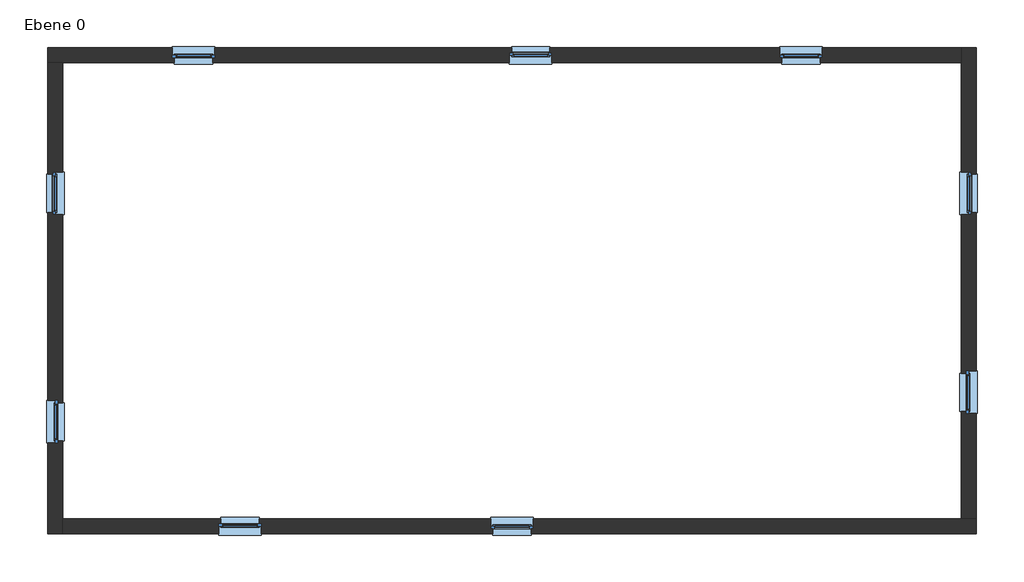
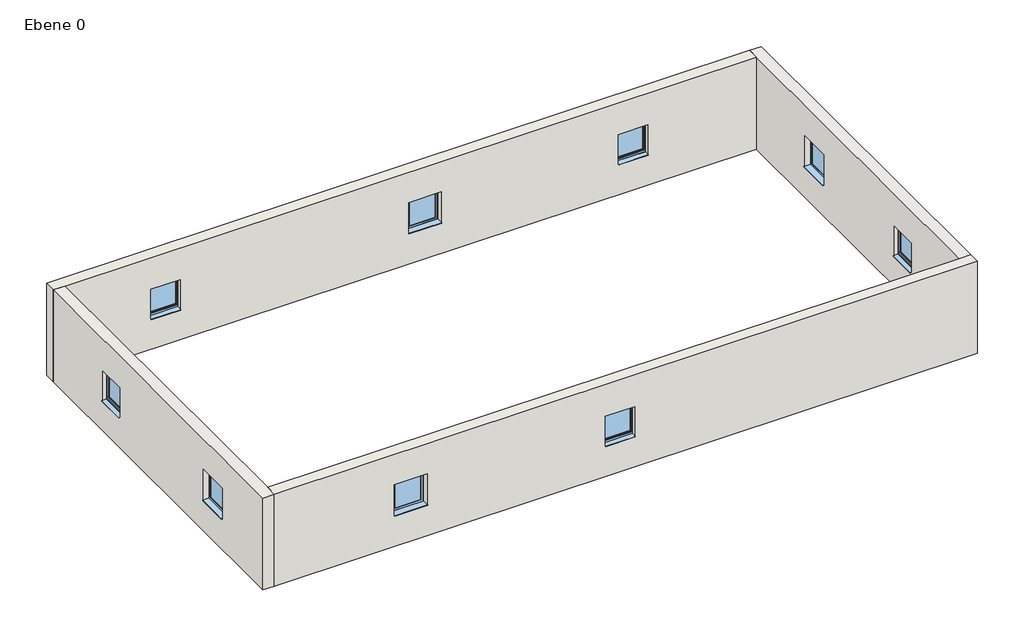
# One storey: 9 windows, 4 walls.
"""IFC4 building model written with IfcOpenShell, lengths in millimetres."""

import ifcopenshell
import ifcopenshell.guid

model = None  # the IFC model being written
_history = None  # IfcOwnerHistory: only IFC2X3 demands one
_inside = {}  # id of a spatial element -> (the spatial element, [elements in it])
_under = {}  # id of a project, library or spatial element -> (it, [spatial elements below it])
_declared = {}  # id of a project -> (the project, [libraries it declares])
_typed = {}  # id of a type object -> (the type object, [elements of that type])
_made_of = {}  # id of a material, layer set ... -> (it, [elements and type objects made of it])


def new_model(schema):
    """Start an empty IFC model of exactly this schema.

    Asked for "IFC4X3", IfcOpenShell would pick the latest addendum, in which some entities
    have other attributes; the version numbers below select the first issue.
    IFC2X3 requires an IfcOwnerHistory on every rooted entity: one is made here for all.
    """
    global model, _history
    if schema == "IFC4X3":
        model = ifcopenshell.file(schema_version=(4, 3, 0, 0))
    else:
        model = ifcopenshell.file(schema=schema)
    _inside.clear()
    _under.clear()
    _declared.clear()
    _typed.clear()
    _made_of.clear()
    _history = None
    if model.schema == "IFC2X3":
        org = make("IfcOrganization", Name="unknown")
        user = make(
            "IfcPersonAndOrganization",
            ThePerson=make("IfcPerson", FamilyName="unknown"),
            TheOrganization=org,
        )
        app = make(
            "IfcApplication",
            ApplicationDeveloper=org,
            Version="unknown",
            ApplicationFullName="unknown",
            ApplicationIdentifier="unknown",
        )
        _history = make(
            "IfcOwnerHistory",
            OwningUser=user,
            OwningApplication=app,
            ChangeAction="ADDED",
            CreationDate=0,
        )
    return model


def make(cls, **values):
    """One entity of the class cls with the attributes given. An attribute that is None is left unset."""
    return model.create_entity(
        cls, **{name: value for name, value in values.items() if value is not None}
    )


def rooted(cls, **values):
    """An entity with a GlobalId (a new one), such as an element, a storey or a relation."""
    return make(cls, GlobalId=ifcopenshell.guid.new(), OwnerHistory=_history, **values)


def si_unit(unit_type, name, prefix=None):
    """IfcSIUnit, for example si_unit("LENGTHUNIT", "METRE", prefix="MILLI")."""
    return make("IfcSIUnit", UnitType=unit_type, Prefix=prefix, Name=name)


def assignment(units):
    """IfcUnitAssignment: the units of a project."""
    return None if units is None else make("IfcUnitAssignment", Units=units)


def point(xyz):
    """IfcCartesianPoint."""
    return None if xyz is None else make("IfcCartesianPoint", Coordinates=xyz)


def direction(xyz):
    """IfcDirection."""
    return None if xyz is None else make("IfcDirection", DirectionRatios=xyz)


def frame(location, z_axis=None, x_axis=None):
    """IfcAxis2Placement3D, a coordinate frame: its origin and axes. An axis left out is left unset."""
    return make(
        "IfcAxis2Placement3D",
        Location=point(location),
        Axis=direction(z_axis),
        RefDirection=direction(x_axis),
    )


def origin():
    """The frame at (0, 0, 0) with its axes left unset."""
    return frame((0.0, 0.0, 0.0))


def place(relative_to, where):
    """IfcLocalPlacement: puts the frame where relative to a parent placement (None: the world)."""
    return make(
        "IfcLocalPlacement", PlacementRelTo=relative_to, RelativePlacement=where
    )


def context(
    kind, dimensions, precision=None, world=None, true_north=None, identifier=None
):
    """IfcGeometricRepresentationContext, for example the 3D "Model" context."""
    return make(
        "IfcGeometricRepresentationContext",
        ContextIdentifier=identifier,
        ContextType=kind,
        CoordinateSpaceDimension=dimensions,
        Precision=precision,
        WorldCoordinateSystem=world,
        TrueNorth=true_north,
    )


def project(units=None, contexts=None):
    """IfcProject with its units and contexts."""
    return rooted(
        "IfcProject",
        Name="project",
        RepresentationContexts=contexts,
        UnitsInContext=assignment(units),
    )


def spatial(cls, under=None, at=None, **own):
    """A site, building, storey or space (cls), placed at a placement, below another one or the project."""
    s = rooted(cls, ObjectPlacement=at, **own)
    if under is not None:
        _under.setdefault(under.id(), (under, []))[1].append(s)
    return s


def polyline(points):
    """IfcPolyline through the points."""
    return make("IfcPolyline", Points=[point(p) for p in points])


def outline(outer, holes=None, kind="AREA"):
    """IfcArbitraryClosedProfileDef: a profile drawn as a closed curve; with holes, ...WithVoids."""
    if holes is None:
        return make("IfcArbitraryClosedProfileDef", ProfileType=kind, OuterCurve=outer)
    return make(
        "IfcArbitraryProfileDefWithVoids",
        ProfileType=kind,
        OuterCurve=outer,
        InnerCurves=holes,
    )


def extrude(swept, where, along, depth):
    """IfcExtrudedAreaSolid: the profile swept, set in the frame where, extruded along a direction by depth."""
    return make(
        "IfcExtrudedAreaSolid",
        SweptArea=swept,
        Position=where,
        ExtrudedDirection=direction(along),
        Depth=depth,
    )


def faces_of(points, faces, orient=None, outer=None):
    """IfcFace entities. A face is a list of loops; a loop is a list of indices into points, from 0.

    orient and outer hold one flag for each loop. By default every Orientation is true, the
    first loop of a face is its IfcFaceOuterBound and the others are IfcFaceBound.
    """
    made = []
    for i, loops in enumerate(faces):
        bounds = []
        for j, loop in enumerate(loops):
            is_outer = j == 0 if outer is None else outer[i][j]
            bounds.append(
                make(
                    "IfcFaceOuterBound" if is_outer else "IfcFaceBound",
                    Bound=make("IfcPolyLoop", Polygon=[points[k] for k in loop]),
                    Orientation=True if orient is None else orient[i][j],
                )
            )
        made.append(make("IfcFace", Bounds=bounds))
    return made


def faceted_brep(points, faces, orient=None, outer=None, voids=None):
    """IfcFacetedBrep: a solid bounded by flat faces; with voids (closed shells), ...WithVoids."""
    shared = [point(p) for p in points]
    hull = make("IfcClosedShell", CfsFaces=faces_of(shared, faces, orient, outer))
    if voids is None:
        return make("IfcFacetedBrep", Outer=hull)
    return make(
        "IfcFacetedBrepWithVoids",
        Outer=hull,
        Voids=[
            make(cls, CfsFaces=faces_of(shared, fs, o, b)) for cls, fs, o, b in voids
        ],
    )


def shape(context_of_items, identifier, shape_type, items):
    """IfcShapeRepresentation: the items that make up one representation, for example the "Body"."""
    return make(
        "IfcShapeRepresentation",
        ContextOfItems=context_of_items,
        RepresentationIdentifier=identifier,
        RepresentationType=shape_type,
        Items=items,
    )


def source(mapping_origin, context_of_items, identifier, shape_type, items):
    """IfcRepresentationMap: a shape defined once, which mapped items show again and again."""
    return make(
        "IfcRepresentationMap",
        MappingOrigin=mapping_origin,
        MappedRepresentation=shape(context_of_items, identifier, shape_type, items),
    )


def transform(
    local_origin,
    x_axis=None,
    y_axis=None,
    z_axis=None,
    scale=None,
    scale2=None,
    scale3=None,
    uniform=True,
):
    """IfcCartesianTransformationOperator3D, or its non-uniform kind. x_axis, y_axis, z_axis: its Axis1, 2, 3."""
    if uniform:
        return make(
            "IfcCartesianTransformationOperator3D",
            Axis1=direction(x_axis),
            Axis2=direction(y_axis),
            LocalOrigin=point(local_origin),
            Scale=scale,
            Axis3=direction(z_axis),
        )
    return make(
        "IfcCartesianTransformationOperator3DnonUniform",
        Axis1=direction(x_axis),
        Axis2=direction(y_axis),
        LocalOrigin=point(local_origin),
        Scale=scale,
        Axis3=direction(z_axis),
        Scale2=scale2,
        Scale3=scale3,
    )


def mapped(mapping_source, mapping_target):
    """IfcMappedItem: shows the shape of a source again, moved by a transform."""
    return make(
        "IfcMappedItem", MappingSource=mapping_source, MappingTarget=mapping_target
    )


def made_of(thing, what):
    """Note that an element or type object is made of a material, layer set ...; save() writes the relation."""
    if what is not None:
        _made_of.setdefault(what.id(), (what, []))[1].append(thing)
    return thing


def element(
    cls,
    number,
    at=None,
    inside=None,
    cuts=None,
    type_object=None,
    material=None,
    context=None,
    identifier="Body",
    shape_type=None,
    held_by="IfcProductDefinitionShape",
    body=None,
    shapes=None,
    **own,
):
    """One element of the class cls, such as IfcWall. Its Tag is "e" and its number.

    at: its placement. inside: the storey or other place that contains it. cuts: it is an
    opening in that element (IfcRelVoidsElement). A single representation is given by context,
    identifier, shape_type and body (its items); several are given by shapes. held_by: the class
    of the entity that holds the representations. save() writes the other relations.
    """
    e = rooted(cls, Tag="e%d" % number, ObjectPlacement=at, **own)
    if body is not None:
        shapes = [shape(context, identifier, shape_type, body)]
    if shapes is not None:
        e.Representation = make(held_by, Representations=shapes)
    if inside is not None:
        _inside.setdefault(inside.id(), (inside, []))[1].append(e)
    if cuts is not None:
        rooted(
            "IfcRelVoidsElement", RelatingBuildingElement=cuts, RelatedOpeningElement=e
        )
    if type_object is not None:
        _typed.setdefault(type_object.id(), (type_object, []))[1].append(e)
    return made_of(e, material)


def aggregate(whole, parts):
    """IfcRelAggregates: a whole, such as a stair, and the parts it consists of."""
    return rooted("IfcRelAggregates", RelatingObject=whole, RelatedObjects=parts)


def save(model, path):
    """Write the relations noted so far, then the file.

    IfcRelAggregates (storeys below a building ...), IfcRelContainedInSpatialStructure (elements
    in a storey), IfcRelDefinesByType, IfcRelAssociatesMaterial and IfcRelDeclares: one each for
    every whole, place, type object, material and project.
    """
    for whole, parts in _under.values():
        aggregate(whole, parts)
    for where, things in _inside.values():
        rooted(
            "IfcRelContainedInSpatialStructure",
            RelatedElements=things,
            RelatingStructure=where,
        )
    for kind, things in _typed.values():
        rooted("IfcRelDefinesByType", RelatedObjects=things, RelatingType=kind)
    for what, things in _made_of.values():
        rooted("IfcRelAssociatesMaterial", RelatedObjects=things, RelatingMaterial=what)
    for by, libraries in _declared.values():
        rooted("IfcRelDeclares", RelatingContext=by, RelatedDefinitions=libraries)
    model.write(path)


def window_1_01_x_1_01_b7243dc8(model_context):
    return source(origin(), model_context, "Body", "SolidModel", [
        extrude(outline(polyline([(-525.0, -210.0), (-525.0, 0.0), (485.0, 0.0), (485.0, -210.0), (-525.0, -210.0)])), frame((0.0, 0.0, 1005.0), z_axis=(0.0, 0.0, 1.0), x_axis=(1.0, 0.0, 0.0)), (0.0, 0.0, 1.0), 15.0),
        extrude(outline(polyline([(375.0, -15.0), (-415.0, -15.0), (-415.0, 15.0), (375.0, 15.0), (375.0, -15.0)])), frame((0.0, 0.0, 1110.0), z_axis=(0.0, 0.0, 1.0), x_axis=(1.0, 0.0, 0.0)), (0.0, 0.0, 1.0), 790.0),
        extrude(outline(polyline([(70.0221543, 1020.0), (210.0, 1000.0), (210.0, 990.0), (208.0, 990.0), (208.0, 998.3604634), (69.8240723, 1018.0), (60.0, 1018.0), (60.0, 1020.0), (70.0221543, 1020.0)])), frame((-475.0, 0.0, 0.0), z_axis=(1.0, 0.0, 0.0), x_axis=(0.0, 1.0, 0.0)), (0.0, 0.0, 1.0), 910.0),
        extrude(outline(polyline([(2010.0, 485.0), (2010.0, -525.0), (1000.0, -525.0), (1000.0, 485.0), (2010.0, 485.0)]), holes=[polyline([(1930.0, 405.0), (1080.0, 405.0), (1080.0, -445.0), (1930.0, -445.0), (1930.0, 405.0)])]), frame((0.0, 0.0, 0.0), z_axis=(0.0, 1.0, 0.0), x_axis=(0.0, 0.0, 1.0)), (0.0, 0.0, 1.0), 60.0),
        faceted_brep([(435.0, 0.0, 1960.0), (435.0, -30.0, 1960.0), (435.0, -30.0, 1050.0), (435.0, 0.0, 1050.0), (-475.0, -30.0, 1960.0), (-475.0, -30.0, 1050.0), (375.0, -30.0, 1110.0), (-415.0, -30.0, 1110.0), (-415.0, -30.0, 1900.0), (375.0, -30.0, 1900.0), (-475.0, 0.0, 1050.0), (-475.0, 0.0, 1960.0), (405.0, 0.0, 1930.0), (-445.0, 0.0, 1930.0), (-445.0, 0.0, 1080.0), (405.0, 0.0, 1080.0), (405.0, 30.0, 1930.0), (405.0, 30.0, 1080.0), (-445.0, 30.0, 1080.0), (-445.0, 30.0, 1930.0), (375.0, 30.0, 1900.0), (-415.0, 30.0, 1900.0), (-415.0, 30.0, 1110.0), (375.0, 30.0, 1110.0)], [[[0, 1, 2, 3]], [[1, 4, 5, 2], [6, 7, 8, 9]], [[3, 2, 5, 10]], [[3, 10, 11, 0], [12, 13, 14, 15]], [[16, 12, 15, 17]], [[17, 15, 14, 18]], [[17, 18, 19, 16], [20, 21, 22, 23]], [[9, 20, 23, 6]], [[6, 23, 22, 7]], [[10, 5, 4, 11]], [[18, 14, 13, 19]], [[7, 22, 21, 8]], [[11, 4, 1, 0]], [[19, 13, 12, 16]], [[8, 21, 20, 9]]]),
    ])


model = new_model("IFC4")

# Units and contexts
model_context = context("Model", 3, world=origin())
ifc_project = project(units=[si_unit("LENGTHUNIT", "METRE", prefix="MILLI")], contexts=[model_context])

# Site, building, storey
site = spatial("IfcSite", under=ifc_project)
building = spatial("IfcBuilding", under=site)
storey = spatial("IfcBuildingStorey", under=building, Name="Ebene 0", Elevation=0.0)

# Walls
placement = place(None, origin())
element("IfcWall", 1, ObjectType="MW 24.0 WD 12.0", at=placement, inside=storey, context=model_context, shape_type="Brep", body=[
    faceted_brep([(-13369.6797169, 6985.6067473, 0.0), (-13009.6797169, 6985.6067473, 0.0), (8330.3202831, 6985.6067473, 0.0), (8330.3202831, 6985.6067473, 3000.0), (-13009.6797169, 6985.6067473, 3000.0), (-13369.6797169, 6985.6067473, 3000.0), (-10359.6797169, 6985.6067473, 1960.0), (-9449.6797169, 6985.6067473, 1960.0), (-9449.6797169, 6985.6067473, 1000.0), (-10359.6797169, 6985.6067473, 1000.0), (-1389.6797169, 6985.6067473, 1000.0), (-2399.6797169, 6985.6067473, 1000.0), (-2399.6797169, 6985.6067473, 2010.0), (-1389.6797169, 6985.6067473, 2010.0), (4070.3202831, 6985.6067473, 1960.0), (4980.3202831, 6985.6067473, 1960.0), (4980.3202831, 6985.6067473, 1000.0), (4070.3202831, 6985.6067473, 1000.0), (-13369.6797169, 7345.6067473, 0.0), (-13369.6797169, 7345.6067473, 3000.0), (8330.3202831, 7345.6067473, 3000.0), (8330.3202831, 7345.6067473, 0.0), (-10409.6797169, 7345.6067473, 1000.0), (-9399.6797169, 7345.6067473, 1000.0), (-9399.6797169, 7345.6067473, 2010.0), (-10409.6797169, 7345.6067473, 2010.0), (-1439.6797169, 7345.6067473, 1960.0), (-2349.6797169, 7345.6067473, 1960.0), (-2349.6797169, 7345.6067473, 1000.0), (-1439.6797169, 7345.6067473, 1000.0), (4020.3202831, 7345.6067473, 1000.0), (5030.3202831, 7345.6067473, 1000.0), (5030.3202831, 7345.6067473, 2010.0), (4020.3202831, 7345.6067473, 2010.0), (-10359.6797169, 7105.6067473, 1960.0), (-9449.6797169, 7105.6067473, 1960.0), (-9449.6797169, 7105.6067473, 1000.0), (-10359.6797169, 7105.6067473, 1000.0), (-9399.6797169, 7105.6067473, 1000.0), (-10409.6797169, 7105.6067473, 1000.0), (-9399.6797169, 7105.6067473, 2010.0), (-10409.6797169, 7105.6067473, 2010.0), (-1439.6797169, 7225.6067473, 1960.0), (-2349.6797169, 7225.6067473, 1960.0), (-2349.6797169, 7225.6067473, 1000.0), (-1439.6797169, 7225.6067473, 1000.0), (-2399.6797169, 7225.6067473, 1000.0), (-1389.6797169, 7225.6067473, 1000.0), (-2399.6797169, 7225.6067473, 2010.0), (-1389.6797169, 7225.6067473, 2010.0), (4070.3202831, 7105.6067473, 1960.0), (4980.3202831, 7105.6067473, 1960.0), (4980.3202831, 7105.6067473, 1000.0), (4070.3202831, 7105.6067473, 1000.0), (5030.3202831, 7105.6067473, 1000.0), (4020.3202831, 7105.6067473, 1000.0), (5030.3202831, 7105.6067473, 2010.0), (4020.3202831, 7105.6067473, 2010.0)], [[[0, 1, 2, 3, 4, 5], [6, 7, 8, 9], [10, 11, 12, 13], [14, 15, 16, 17]], [[18, 19, 20, 21], [22, 23, 24, 25], [26, 27, 28, 29], [30, 31, 32, 33]], [[2, 1, 0, 18, 21]], [[5, 4, 3, 20, 19]], [[0, 5, 19, 18]], [[3, 2, 21, 20]], [[6, 34, 35, 7]], [[7, 35, 36, 8]], [[34, 6, 9, 37]], [[8, 36, 38, 23, 22, 39, 37, 9]], [[40, 41, 25, 24]], [[41, 39, 22, 25]], [[41, 40, 38, 36, 35, 34, 37, 39]], [[38, 40, 24, 23]], [[26, 42, 43, 27]], [[27, 43, 44, 28]], [[42, 26, 29, 45]], [[28, 44, 46, 11, 10, 47, 45, 29]], [[48, 49, 13, 12]], [[49, 47, 10, 13]], [[49, 48, 46, 44, 43, 42, 45, 47]], [[46, 48, 12, 11]], [[14, 50, 51, 15]], [[15, 51, 52, 16]], [[50, 14, 17, 53]], [[16, 52, 54, 31, 30, 55, 53, 17]], [[56, 57, 33, 32]], [[57, 55, 30, 33]], [[57, 56, 54, 52, 51, 50, 53, 55]], [[54, 56, 32, 31]]]),
])
element("IfcWall", 2, ObjectType="MW 24.0 WD 12.0", at=placement, inside=storey, context=model_context, shape_type="Brep", body=[
    faceted_brep([(-13009.6797169, -4214.3932527, 0.0), (-13009.6797169, -3854.3932527, 0.0), (-13009.6797169, 6985.6067473, 0.0), (-13009.6797169, 6985.6067473, 3000.0), (-13009.6797169, -3854.3932527, 3000.0), (-13009.6797169, -4214.3932527, 3000.0), (-13009.6797169, -2004.3932527, 1960.0), (-13009.6797169, -1094.3932527, 1960.0), (-13009.6797169, -1094.3932527, 1000.0), (-13009.6797169, -2004.3932527, 1000.0), (-13009.6797169, 4385.6067473, 1000.0), (-13009.6797169, 3375.6067473, 1000.0), (-13009.6797169, 3375.6067473, 2010.0), (-13009.6797169, 4385.6067473, 2010.0), (-13369.6797169, -4214.3932527, 0.0), (-13369.6797169, -4214.3932527, 3000.0), (-13369.6797169, 6985.6067473, 3000.0), (-13369.6797169, 6985.6067473, 0.0), (-13369.6797169, -2054.3932527, 1000.0), (-13369.6797169, -1044.3932527, 1000.0), (-13369.6797169, -1044.3932527, 2010.0), (-13369.6797169, -2054.3932527, 2010.0), (-13369.6797169, 4335.6067473, 1960.0), (-13369.6797169, 3425.6067473, 1960.0), (-13369.6797169, 3425.6067473, 1000.0), (-13369.6797169, 4335.6067473, 1000.0), (-13129.6797169, -2004.3932527, 1960.0), (-13129.6797169, -1094.3932527, 1960.0), (-13129.6797169, -1094.3932527, 1000.0), (-13129.6797169, -2004.3932527, 1000.0), (-13129.6797169, -1044.3932527, 1000.0), (-13129.6797169, -2054.3932527, 1000.0), (-13129.6797169, -1044.3932527, 2010.0), (-13129.6797169, -2054.3932527, 2010.0), (-13249.6797169, 4335.6067473, 1960.0), (-13249.6797169, 3425.6067473, 1960.0), (-13249.6797169, 3425.6067473, 1000.0), (-13249.6797169, 4335.6067473, 1000.0), (-13249.6797169, 3375.6067473, 1000.0), (-13249.6797169, 4385.6067473, 1000.0), (-13249.6797169, 3375.6067473, 2010.0), (-13249.6797169, 4385.6067473, 2010.0)], [[[0, 1, 2, 3, 4, 5], [6, 7, 8, 9], [10, 11, 12, 13]], [[14, 15, 16, 17], [18, 19, 20, 21], [22, 23, 24, 25]], [[2, 1, 0, 14, 17]], [[5, 4, 3, 16, 15]], [[0, 5, 15, 14]], [[3, 2, 17, 16]], [[6, 26, 27, 7]], [[7, 27, 28, 8]], [[26, 6, 9, 29]], [[8, 28, 30, 19, 18, 31, 29, 9]], [[32, 33, 21, 20]], [[33, 31, 18, 21]], [[33, 32, 30, 28, 27, 26, 29, 31]], [[30, 32, 20, 19]], [[22, 34, 35, 23]], [[23, 35, 36, 24]], [[34, 22, 25, 37]], [[24, 36, 38, 11, 10, 39, 37, 25]], [[40, 41, 13, 12]], [[41, 39, 10, 13]], [[41, 40, 38, 36, 35, 34, 37, 39]], [[38, 40, 12, 11]]]),
])
element("IfcWall", 3, ObjectType="MW 24.0 WD 12.0", at=placement, inside=storey, context=model_context, shape_type="Brep", body=[
    faceted_brep([(8690.3202831, -3854.3932527, 0.0), (8330.3202831, -3854.3932527, 0.0), (-13009.6797169, -3854.3932527, 0.0), (-13009.6797169, -3854.3932527, 3000.0), (8330.3202831, -3854.3932527, 3000.0), (8690.3202831, -3854.3932527, 3000.0), (-2844.6797169, -3854.3932527, 1000.0), (-1834.6797169, -3854.3932527, 1000.0), (-1834.6797169, -3854.3932527, 2010.0), (-2844.6797169, -3854.3932527, 2010.0), (-8349.6797169, -3854.3932527, 1960.0), (-9259.6797169, -3854.3932527, 1960.0), (-9259.6797169, -3854.3932527, 1000.0), (-8349.6797169, -3854.3932527, 1000.0), (8690.3202831, -4214.3932527, 0.0), (8690.3202831, -4214.3932527, 3000.0), (-13009.6797169, -4214.3932527, 3000.0), (-13009.6797169, -4214.3932527, 0.0), (-2794.6797169, -4214.3932527, 1960.0), (-1884.6797169, -4214.3932527, 1960.0), (-1884.6797169, -4214.3932527, 1000.0), (-2794.6797169, -4214.3932527, 1000.0), (-8299.6797169, -4214.3932527, 1000.0), (-9309.6797169, -4214.3932527, 1000.0), (-9309.6797169, -4214.3932527, 2010.0), (-8299.6797169, -4214.3932527, 2010.0), (-2794.6797169, -4094.3932527, 1960.0), (-1884.6797169, -4094.3932527, 1960.0), (-1884.6797169, -4094.3932527, 1000.0), (-2794.6797169, -4094.3932527, 1000.0), (-1834.6797169, -4094.3932527, 1000.0), (-2844.6797169, -4094.3932527, 1000.0), (-1834.6797169, -4094.3932527, 2010.0), (-2844.6797169, -4094.3932527, 2010.0), (-8349.6797169, -3974.3932527, 1960.0), (-9259.6797169, -3974.3932527, 1960.0), (-9259.6797169, -3974.3932527, 1000.0), (-8349.6797169, -3974.3932527, 1000.0), (-9309.6797169, -3974.3932527, 1000.0), (-8299.6797169, -3974.3932527, 1000.0), (-9309.6797169, -3974.3932527, 2010.0), (-8299.6797169, -3974.3932527, 2010.0)], [[[0, 1, 2, 3, 4, 5], [6, 7, 8, 9], [10, 11, 12, 13]], [[14, 15, 16, 17], [18, 19, 20, 21], [22, 23, 24, 25]], [[2, 1, 0, 14, 17]], [[5, 4, 3, 16, 15]], [[0, 5, 15, 14]], [[3, 2, 17, 16]], [[18, 26, 27, 19]], [[19, 27, 28, 20]], [[26, 18, 21, 29]], [[20, 28, 30, 7, 6, 31, 29, 21]], [[32, 33, 9, 8]], [[33, 31, 6, 9]], [[33, 32, 30, 28, 27, 26, 29, 31]], [[30, 32, 8, 7]], [[10, 34, 35, 11]], [[11, 35, 36, 12]], [[34, 10, 13, 37]], [[12, 36, 38, 23, 22, 39, 37, 13]], [[40, 41, 25, 24]], [[41, 39, 22, 25]], [[41, 40, 38, 36, 35, 34, 37, 39]], [[38, 40, 24, 23]]]),
])
element("IfcWall", 4, ObjectType="MW 24.0 WD 12.0", at=placement, inside=storey, context=model_context, shape_type="Brep", body=[
    faceted_brep([(8330.3202831, 7345.6067473, 0.0), (8330.3202831, 6985.6067473, 0.0), (8330.3202831, -3854.3932527, 0.0), (8330.3202831, -3854.3932527, 3000.0), (8330.3202831, 6985.6067473, 3000.0), (8330.3202831, 7345.6067473, 3000.0), (8330.3202831, 3375.6067473, 1000.0), (8330.3202831, 4385.6067473, 1000.0), (8330.3202831, 4385.6067473, 2010.0), (8330.3202831, 3375.6067473, 2010.0), (8330.3202831, -394.3932527, 1960.0), (8330.3202831, -1304.3932527, 1960.0), (8330.3202831, -1304.3932527, 1000.0), (8330.3202831, -394.3932527, 1000.0), (8690.3202831, 7345.6067473, 0.0), (8690.3202831, 7345.6067473, 3000.0), (8690.3202831, -3854.3932527, 3000.0), (8690.3202831, -3854.3932527, 0.0), (8690.3202831, 3425.6067473, 1960.0), (8690.3202831, 4335.6067473, 1960.0), (8690.3202831, 4335.6067473, 1000.0), (8690.3202831, 3425.6067473, 1000.0), (8690.3202831, -344.3932527, 1000.0), (8690.3202831, -1354.3932527, 1000.0), (8690.3202831, -1354.3932527, 2010.0), (8690.3202831, -344.3932527, 2010.0), (8570.3202831, 3425.6067473, 1960.0), (8570.3202831, 4335.6067473, 1960.0), (8570.3202831, 4335.6067473, 1000.0), (8570.3202831, 3425.6067473, 1000.0), (8570.3202831, 4385.6067473, 1000.0), (8570.3202831, 3375.6067473, 1000.0), (8570.3202831, 4385.6067473, 2010.0), (8570.3202831, 3375.6067473, 2010.0), (8450.3202831, -394.3932527, 1960.0), (8450.3202831, -1304.3932527, 1960.0), (8450.3202831, -1304.3932527, 1000.0), (8450.3202831, -394.3932527, 1000.0), (8450.3202831, -1354.3932527, 1000.0), (8450.3202831, -344.3932527, 1000.0), (8450.3202831, -1354.3932527, 2010.0), (8450.3202831, -344.3932527, 2010.0)], [[[0, 1, 2, 3, 4, 5], [6, 7, 8, 9], [10, 11, 12, 13]], [[14, 15, 16, 17], [18, 19, 20, 21], [22, 23, 24, 25]], [[2, 1, 0, 14, 17]], [[5, 4, 3, 16, 15]], [[0, 5, 15, 14]], [[3, 2, 17, 16]], [[18, 26, 27, 19]], [[19, 27, 28, 20]], [[26, 18, 21, 29]], [[20, 28, 30, 7, 6, 31, 29, 21]], [[32, 33, 9, 8]], [[33, 31, 6, 9]], [[33, 32, 30, 28, 27, 26, 29, 31]], [[30, 32, 8, 7]], [[10, 34, 35, 11]], [[11, 35, 36, 12]], [[34, 10, 13, 37]], [[12, 36, 38, 23, 22, 39, 37, 13]], [[40, 41, 25, 24]], [[41, 39, 22, 25]], [[41, 40, 38, 36, 35, 34, 37, 39]], [[38, 40, 24, 23]]]),
])

# Windows
window_1_01_x_1_01_shape = window_1_01_x_1_01_b7243dc8(model_context)
element("IfcWindow", 5, ObjectType="Fenster 1-flg - Anschlag : 1.01 x 1.01", at=placement, inside=storey, context=model_context, shape_type="MappedRepresentation", body=[
    mapped(window_1_01_x_1_01_shape, transform((-1874.6797169, 7165.6067473, 0.0), x_axis=(1.0, 0.0, 0.0), y_axis=(0.0, 1.0, 0.0), z_axis=(0.0, 0.0, 1.0))),
])
element("IfcWindow", 6, ObjectType="Fenster 1-flg - Anschlag : 1.01 x 1.01", at=placement, inside=storey, context=model_context, shape_type="MappedRepresentation", body=[
    mapped(window_1_01_x_1_01_shape, transform((8510.3202831, 3860.6067473, 0.0), x_axis=(0.0, -1.0, 0.0), y_axis=(1.0, 0.0, 0.0), z_axis=(0.0, 0.0, 1.0))),
])
element("IfcWindow", 7, ObjectType="Fenster 1-flg - Anschlag : 1.01 x 1.01", at=placement, inside=storey, context=model_context, shape_type="MappedRepresentation", body=[
    mapped(window_1_01_x_1_01_shape, transform((-2359.6797169, -4034.3932527, 0.0), x_axis=(-1.0, 0.0, 0.0), y_axis=(0.0, -1.0, 0.0), z_axis=(0.0, 0.0, 1.0))),
])
element("IfcWindow", 8, ObjectType="Fenster 1-flg - Anschlag : 1.01 x 1.01", at=placement, inside=storey, context=model_context, shape_type="MappedRepresentation", body=[
    mapped(window_1_01_x_1_01_shape, transform((-13189.6797169, 3900.6067473, 0.0), x_axis=(0.0, 1.0, 0.0), y_axis=(-1.0, 0.0, 0.0), z_axis=(0.0, 0.0, 1.0))),
])
element("IfcWindow", 9, ObjectType="Fenster 1-flg - Anschlag : 1.01 x 1.01", at=placement, inside=storey, context=model_context, shape_type="MappedRepresentation", body=[
    mapped(window_1_01_x_1_01_shape, transform((-9924.6797169, 7165.6067473, 0.0), x_axis=(-1.0, 0.0, 0.0), y_axis=(0.0, -1.0, 0.0), z_axis=(0.0, 0.0, 1.0))),
])
element("IfcWindow", 10, ObjectType="Fenster 1-flg - Anschlag : 1.01 x 1.01", at=placement, inside=storey, context=model_context, shape_type="MappedRepresentation", body=[
    mapped(window_1_01_x_1_01_shape, transform((4505.3202831, 7165.6067473, 0.0), x_axis=(-1.0, 0.0, 0.0), y_axis=(0.0, -1.0, 0.0), z_axis=(0.0, 0.0, 1.0))),
])
element("IfcWindow", 11, ObjectType="Fenster 1-flg - Anschlag : 1.01 x 1.01", at=placement, inside=storey, context=model_context, shape_type="MappedRepresentation", body=[
    mapped(window_1_01_x_1_01_shape, transform((8510.3202831, -829.3932527, 0.0), x_axis=(0.0, 1.0, 0.0), y_axis=(-1.0, 0.0, 0.0), z_axis=(0.0, 0.0, 1.0))),
])
element("IfcWindow", 12, ObjectType="Fenster 1-flg - Anschlag : 1.01 x 1.01", at=placement, inside=storey, context=model_context, shape_type="MappedRepresentation", body=[
    mapped(window_1_01_x_1_01_shape, transform((-8784.6797169, -4034.3932527, 0.0), x_axis=(1.0, 0.0, 0.0), y_axis=(0.0, 1.0, 0.0), z_axis=(0.0, 0.0, 1.0))),
])
element("IfcWindow", 13, ObjectType="Fenster 1-flg - Anschlag : 1.01 x 1.01", at=placement, inside=storey, context=model_context, shape_type="MappedRepresentation", body=[
    mapped(window_1_01_x_1_01_shape, transform((-13189.6797169, -1569.3932527, 0.0), x_axis=(0.0, -1.0, 0.0), y_axis=(1.0, 0.0, 0.0), z_axis=(0.0, 0.0, 1.0))),
])

save(model, "model.ifc")

# Revit data of these elements
# Project information
#   Projektausgabedatum = "Projekt Datum"
#   Projektstatus = "Projektstatus"
#   Kundenname = "Bauherr"
#   Projektadresse = "Projektadresse"
#   Projektname = "Projektname"
#   Projektnummer = "Projektnummer"
#   Verfasser Firma 1 = "Firma 1"
#   Verfasser Firma 2 = "Firma 2"
#   Verfasser PLZ Ort = "PLZ Ort"
#   Verfasser Strasse = "Strasse"
#   Verfasser Telefon = "Telefon"
#   Verfasser Telefax = "Telefax"
#   Verfasser eMail = "E-Mail"
# Type "MW 24.0 WD 12.0"
#   Type Comments = "Mehrschaliges Mauerwerk"
#   Description = "Mauerwerk 24.0 cm, Wärmedämmung 12.0 cm"
#   Width = 0.360 m
#   Layers, outside or top first: 0.120 m "Wärmedämmung - Hart" (function 3); 0.240 m "Mauerwerk - Ziegel, verputzt" (function 1)
# Type "Fenster 1-flg - Anschlag : 1.01 x 1.01"
#   Type Mark = "47"
#   Operation = "SinglePanel"
#   Keynote = "16.05.01"
#   Construction Type Id = "GSP4R"
#   Analytic Construction = "1/8 Zoll Pilkington-Verglasung einfach"
#   Visual Light Transmittance = 0.9
#   Thermal Resistance (R) = 0.1491 (m²·K)/W
#   Solar Heat Gain Coefficient = 0.86
#   Anschlagsbreite seitlich = 0.050 m
#   Rough Width = 1.010 m
#   Rough Height = 1.010 m
#   Heat Transfer Coefficient (U) = 6.7069 W/(m²·K)
#   Rahmentiefe = 0.060 m
#   Rahmenhöhe unten = 0.080 m
#   Rahmenhöhe oben = 0.080 m
#   Rahmenbreite = 0.080 m
#   Height = 1.010 m
#   Flügeltiefe = 0.060 m
#   Flügelbreite = 0.060 m
#   Einbautiefe (von außen) [instance default] = 0.120 m
#   Width = 1.010 m
#   Anschlagsbreite oben = 0.050 m
#   Klappflügel [instance default] = no
#   Öffnungsrichtung oben [instance default] = yes
#   Öffnungsrichtung in Draufsicht anzeigen [instance default] = no
#   Drehflügel [instance default] = yes
#   Rahmen [instance default] = none
#   Glas [instance default] = none
#   Flügel [instance default] = none
#   Fensterbank innen [instance default] = none
#   Fensterbank außen [instance default] = none
#   Wall Closure = (empty or 0)
# Elements 1, 2, 3, 4 (IfcWall, "MW 24.0 WD 12.0")
#   Top Offset = 0.000 m
#   Base Offset = 0.000 m
#   wall height = 3.000 m
#   Phase Created = Phase 1
#   Base Constraint = Ebene 0
#   Top Constraint = Ebene 1
#   Materials on its faces: "Standard - Wand", "Wärmedämmung - Hart", "Mauerwerk - Ziegel, verputzt"
# Element 5 (IfcWindow, "Fenster 1-flg - Anschlag : 1.01 x 1.01")
#   Mark = "2"
#   Einbautiefe (von außen) = 0.120 m
#   Öffnungsrichtung oben = yes
#   Öffnungsrichtung in Draufsicht anzeigen = no
#   Klappflügel = no
#   Drehflügel = yes
#   Rahmen = none
#   Glas = none
#   Flügel = none
#   Fensterbank innen = none
#   Fensterbank außen = none
#   Phase Created = Phase 1
#   Materials on its faces: "Kunststoff - Weiß", "Holz - Birke", "Glas"
# Element 6 (IfcWindow, "Fenster 1-flg - Anschlag : 1.01 x 1.01")
#   Mark = "4"
#   Einbautiefe (von außen) = 0.120 m
#   Öffnungsrichtung oben = yes
#   Öffnungsrichtung in Draufsicht anzeigen = no
#   Klappflügel = no
#   Drehflügel = yes
#   Rahmen = none
#   Glas = none
#   Flügel = none
#   Fensterbank innen = none
#   Fensterbank außen = none
#   Phase Created = Phase 1
#   Materials on its faces: "Kunststoff - Weiß", "Holz - Birke", "Glas"
# Element 7 (IfcWindow, "Fenster 1-flg - Anschlag : 1.01 x 1.01")
#   Mark = "6"
#   Einbautiefe (von außen) = 0.120 m
#   Öffnungsrichtung oben = yes
#   Öffnungsrichtung in Draufsicht anzeigen = no
#   Klappflügel = no
#   Drehflügel = yes
#   Rahmen = none
#   Glas = none
#   Flügel = none
#   Fensterbank innen = none
#   Fensterbank außen = none
#   Phase Created = Phase 1
#   Materials on its faces: "Kunststoff - Weiß", "Holz - Birke", "Glas"
# Element 8 (IfcWindow, "Fenster 1-flg - Anschlag : 1.01 x 1.01")
#   Mark = "9"
#   Einbautiefe (von außen) = 0.120 m
#   Öffnungsrichtung oben = yes
#   Öffnungsrichtung in Draufsicht anzeigen = no
#   Klappflügel = no
#   Drehflügel = yes
#   Rahmen = none
#   Glas = none
#   Flügel = none
#   Fensterbank innen = none
#   Fensterbank außen = none
#   Phase Created = Phase 1
#   Materials on its faces: "Kunststoff - Weiß", "Holz - Birke", "Glas"
# Element 9 (IfcWindow, "Fenster 1-flg - Anschlag : 1.01 x 1.01")
#   Mark = "1"
#   Einbautiefe (von außen) = 0.120 m
#   Öffnungsrichtung oben = yes
#   Öffnungsrichtung in Draufsicht anzeigen = no
#   Klappflügel = no
#   Drehflügel = yes
#   Rahmen = none
#   Glas = none
#   Flügel = none
#   Fensterbank innen = none
#   Fensterbank außen = none
#   Phase Created = Phase 1
#   Materials on its faces: "Kunststoff - Weiß", "Holz - Birke", "Glas"
# Element 10 (IfcWindow, "Fenster 1-flg - Anschlag : 1.01 x 1.01")
#   Mark = "3"
#   Einbautiefe (von außen) = 0.120 m
#   Öffnungsrichtung oben = yes
#   Öffnungsrichtung in Draufsicht anzeigen = no
#   Klappflügel = no
#   Drehflügel = yes
#   Rahmen = none
#   Glas = none
#   Flügel = none
#   Fensterbank innen = none
#   Fensterbank außen = none
#   Phase Created = Phase 1
#   Materials on its faces: "Kunststoff - Weiß", "Holz - Birke", "Glas"
# Element 11 (IfcWindow, "Fenster 1-flg - Anschlag : 1.01 x 1.01")
#   Mark = "5"
#   Einbautiefe (von außen) = 0.120 m
#   Öffnungsrichtung oben = yes
#   Öffnungsrichtung in Draufsicht anzeigen = no
#   Klappflügel = no
#   Drehflügel = yes
#   Rahmen = none
#   Glas = none
#   Flügel = none
#   Fensterbank innen = none
#   Fensterbank außen = none
#   Phase Created = Phase 1
#   Materials on its faces: "Kunststoff - Weiß", "Holz - Birke", "Glas"
# Element 12 (IfcWindow, "Fenster 1-flg - Anschlag : 1.01 x 1.01")
#   Mark = "7"
#   Einbautiefe (von außen) = 0.120 m
#   Öffnungsrichtung oben = yes
#   Öffnungsrichtung in Draufsicht anzeigen = no
#   Klappflügel = no
#   Drehflügel = yes
#   Rahmen = none
#   Glas = none
#   Flügel = none
#   Fensterbank innen = none
#   Fensterbank außen = none
#   Phase Created = Phase 1
#   Materials on its faces: "Kunststoff - Weiß", "Holz - Birke", "Glas"
# Element 13 (IfcWindow, "Fenster 1-flg - Anschlag : 1.01 x 1.01")
#   Mark = "8"
#   Einbautiefe (von außen) = 0.120 m
#   Öffnungsrichtung oben = yes
#   Öffnungsrichtung in Draufsicht anzeigen = no
#   Klappflügel = no
#   Drehflügel = yes
#   Rahmen = none
#   Glas = none
#   Flügel = none
#   Fensterbank innen = none
#   Fensterbank außen = none
#   Phase Created = Phase 1
#   Materials on its faces: "Kunststoff - Weiß", "Holz - Birke", "Glas"
# Materials
#   "Wärmedämmung - Hart": class "Putz", colour RGB 255 255 255, transparency 0, Description = "Äußere Oberfläche"
#   "Mauerwerk - Ziegel, verputzt": class "Putz", colour RGB 247 247 247, transparency 0, Cost = 0
#   "Standard - Wand": class "Putz", colour RGB 128 128 128, transparency 0, Description = "Äußere Oberfläche"
#   "Kunststoff - Weiß": class "Kunststoff", colour RGB 249 249 249, transparency 0
#   "Holz - Birke": class "Holz", colour RGB 213 164 103, transparency 0
#   "Glas": class "Glas", colour RGB 0 0 255, transparency 0.75, Comments = "Renderdarstellung nicht aktualisiert ", Cost = 0
